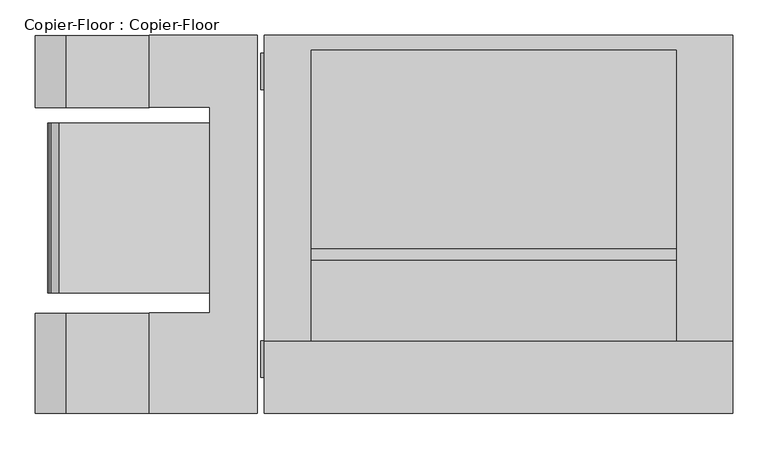
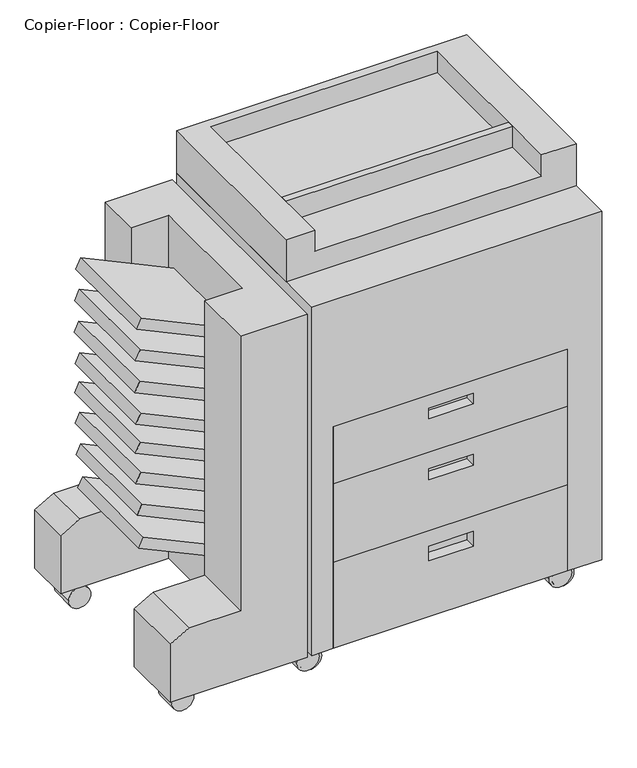
"""IFC4 building model written with IfcOpenShell, lengths in millimetres: proxy geometry, Copier-Floor : Copier-Floor."""

from ifc_helpers import new_model, si_unit, point, frame, frame_2d, origin, place, context, project, spatial, polyline, circle_curve, trimmed, segment, composite_curve, outline, extrude, faceted_brep, source, transform, mapped, element, save


def copier_floor_copier_floor_8d74970a(model_context):
    return source(origin(), model_context, "Body", "SolidModel", [
        extrude(outline(polyline([(358.0987222, -618.0517332), (335.0785044, -628.7862371), (232.9041289, -409.6725817), (260.929928, -409.6725817), (358.0987222, -618.0517332)])), frame((0.0, -72.1685532, 0.0), z_axis=(0.0, 1.0, 0.0), x_axis=(0.0, 0.0, 1.0)), (0.0, 0.0, 1.0), 239.8222339),
        extrude(outline(polyline([(438.9521671, -622.0116402), (415.9319493, -632.7461441), (311.9110388, -409.6725817), (339.9368379, -409.6725817), (438.9521671, -622.0116402)])), frame((0.0, -72.1685532, 0.0), z_axis=(0.0, 1.0, 0.0), x_axis=(0.0, 0.0, 1.0)), (0.0, 0.0, 1.0), 239.8222339),
        extrude(outline(polyline([(516.4459532, -624.7861736), (493.4257355, -635.5206775), (388.1110388, -409.6725817), (416.1368379, -409.6725817), (516.4459532, -624.7861736)])), frame((0.0, -72.1685532, 0.0), z_axis=(0.0, 1.0, 0.0), x_axis=(0.0, 0.0, 1.0)), (0.0, 0.0, 1.0), 239.8222339),
        extrude(outline(polyline([(811.8732774, -625.5671218), (788.8530596, -636.3016256), (683.1742009, -409.6725817), (711.2, -409.6725817), (811.8732774, -625.5671218)])), frame((0.0, -72.1685532, 0.0), z_axis=(0.0, 1.0, 0.0), x_axis=(0.0, 0.0, 1.0)), (0.0, 0.0, 1.0), 239.8222339),
        extrude(outline(polyline([(589.7121876, -625.7577903), (566.6919698, -636.4922942), (460.9242009, -409.6725817), (488.95, -409.6725817), (589.7121876, -625.7577903)])), frame((0.0, -72.1685532, 0.0), z_axis=(0.0, 1.0, 0.0), x_axis=(0.0, 0.0, 1.0)), (0.0, 0.0, 1.0), 239.8222339),
        extrude(outline(polyline([(659.0988749, -624.7642131), (636.0786571, -635.4987169), (530.7742009, -409.6725817), (558.8, -409.6725817), (659.0988749, -624.7642131)])), frame((0.0, -72.1685532, 0.0), z_axis=(0.0, 1.0, 0.0), x_axis=(0.0, 0.0, 1.0)), (0.0, 0.0, 1.0), 239.8222339),
        extrude(outline(polyline([(736.3657716, -627.0521803), (713.3455538, -637.7866841), (606.9742009, -409.6725817), (635.0, -409.6725817), (736.3657716, -627.0521803)])), frame((0.0, -72.1685532, 0.0), z_axis=(0.0, 1.0, 0.0), x_axis=(0.0, 0.0, 1.0)), (0.0, 0.0, 1.0), 239.8222339),
        faceted_brep([(-655.4522418, -242.0310532, 76.2), (-342.5743224, -242.0310532, 76.2), (-342.5743224, -242.0310532, 901.7), (-494.9743224, -242.0310532, 901.7), (-494.9743224, -242.0310532, 241.3), (-612.1273026, -242.0310532, 241.3), (-655.4522418, -242.0310532, 216.2863347), (-655.4522418, 291.3689468, 76.2), (-655.4522418, 291.3689468, 216.2863347), (-612.1273026, 291.3689468, 241.3), (-494.9743224, 291.3689468, 241.3), (-494.9743224, 291.3689468, 901.7), (-342.5743224, 291.3689468, 901.7), (-342.5743224, 291.3689468, 76.2), (-655.4522418, -100.8888364, 76.2), (-409.6725817, -100.8888364, 76.2), (-409.6725817, 189.7689468, 76.2), (-655.4522418, 189.7689468, 76.2), (-494.9743224, 189.7689468, 901.7), (-409.6725817, 189.7689468, 901.7), (-409.6725817, -100.8888364, 901.7), (-494.9743224, -100.8888364, 901.7), (-494.9743224, -100.8888364, 241.3), (-494.9743224, 189.7689468, 241.3), (-612.1273026, -100.8888364, 241.3), (-612.1273026, 189.7689468, 241.3), (-655.4522418, -100.8888364, 216.2863347), (-655.4522418, 189.7689468, 216.2863347)], [[[0, 1, 2, 3, 4, 5, 6]], [[7, 8, 9, 10, 11, 12, 13]], [[1, 0, 14, 15, 16, 17, 7, 13]], [[2, 1, 13, 12]], [[3, 2, 12, 11, 18, 19, 20, 21]], [[4, 3, 21, 22]], [[11, 10, 23, 18]], [[5, 4, 22, 24]], [[10, 9, 25, 23]], [[6, 5, 24, 26]], [[9, 8, 27, 25]], [[0, 6, 26, 14]], [[8, 7, 17, 27]], [[16, 19, 18, 23, 25, 27, 17]], [[20, 15, 14, 26, 24, 22, 21]], [[19, 16, 15, 20]]]),
        faceted_brep([(249.314028, -242.0310532, 472.3553727), (249.314028, -242.0310532, 609.6), (-284.085972, -242.0310532, 609.6), (-284.085972, -242.0310532, 472.3553727), (-66.7741493, -242.0310532, 578.8591447), (34.8258507, -242.0310532, 578.8591447), (34.8258507, -242.0310532, 553.4591447), (-66.7741493, -242.0310532, 553.4591447), (249.314028, -191.2310532, 472.3553727), (-284.085972, -191.2310532, 472.3553727), (-284.085972, -191.2310532, 609.6), (249.314028, -191.2310532, 609.6), (34.8258507, -216.6310532, 578.8591447), (-66.7741493, -216.6310532, 578.8591447), (-66.7741493, -216.6310532, 553.4591447), (34.8258507, -216.6310532, 553.4591447)], [[[0, 1, 2, 3], [4, 5, 6, 7]], [[8, 9, 10, 11]], [[1, 0, 8, 11]], [[2, 1, 11, 10]], [[3, 2, 10, 9]], [[0, 3, 9, 8]], [[12, 13, 14, 15]], [[13, 12, 5, 4]], [[14, 13, 4, 7]], [[15, 14, 7, 6]], [[12, 15, 6, 5]]]),
        faceted_brep([(249.314028, -242.0310532, 283.8723489), (249.314028, -242.0310532, 472.3553727), (-284.085972, -242.0310532, 472.3553727), (-284.085972, -242.0310532, 283.8723489), (-66.7741493, -242.0310532, 432.3774172), (34.8258507, -242.0310532, 432.3774172), (34.8258507, -242.0310532, 406.4), (-66.7741493, -242.0310532, 406.4), (249.314028, -191.2310532, 283.8723489), (-284.085972, -191.2310532, 283.8723489), (-284.085972, -191.2310532, 472.3553727), (249.314028, -191.2310532, 472.3553727), (34.8258507, -216.6310532, 432.3774172), (-66.7741493, -216.6310532, 432.3774172), (-66.7741493, -216.6310532, 406.4), (34.8258507, -216.6310532, 406.4)], [[[0, 1, 2, 3], [4, 5, 6, 7]], [[8, 9, 10, 11]], [[1, 0, 8, 11]], [[2, 1, 11, 10]], [[3, 2, 10, 9]], [[0, 3, 9, 8]], [[12, 13, 14, 15]], [[13, 12, 5, 4]], [[14, 13, 4, 7]], [[15, 14, 7, 6]], [[12, 15, 6, 5]]]),
        faceted_brep([(249.314028, -242.0310532, 76.2), (249.314028, -242.0310532, 283.8723489), (-284.085972, -242.0310532, 283.8723489), (-284.085972, -242.0310532, 76.2), (-66.7741493, -242.0310532, 246.5423898), (34.8258507, -242.0310532, 246.5423898), (34.8258507, -242.0310532, 211.1096445), (-66.7741493, -242.0310532, 211.1096445), (249.314028, -191.2310532, 76.2), (-284.085972, -191.2310532, 76.2), (-284.085972, -191.2310532, 283.8723489), (249.314028, -191.2310532, 283.8723489), (34.8258507, -216.6310532, 246.5423898), (-66.7741493, -216.6310532, 246.5423898), (-66.7741493, -216.6310532, 211.1096445), (34.8258507, -216.6310532, 211.1096445)], [[[0, 1, 2, 3], [4, 5, 6, 7]], [[8, 9, 10, 11]], [[1, 0, 8, 11]], [[2, 1, 11, 10]], [[3, 2, 10, 9]], [[0, 3, 9, 8]], [[12, 13, 14, 15]], [[13, 12, 5, 4]], [[14, 13, 4, 7]], [[15, 14, 7, 6]], [[12, 15, 6, 5]]]),
        faceted_brep([(328.0345418, 291.3689468, 1016.0), (-332.3654582, 291.3689468, 1016.0), (-332.3654582, -139.9052479, 1016.0), (-267.2959958, -139.9052479, 1016.0), (-267.2959958, 271.1108348, 1016.0), (249.314028, 271.1108348, 1016.0), (249.314028, -139.9052479, 1016.0), (328.0345418, -139.9052479, 1016.0), (328.0345418, 291.3689468, 914.4), (328.0345418, -139.9052479, 914.4), (-332.3654582, -139.9052479, 914.4), (-332.3654582, 291.3689468, 914.4), (249.314028, -139.9052479, 965.2), (-267.2959958, -139.9052479, 965.2), (249.314028, 271.1108348, 965.2), (-267.2959958, 271.1108348, 965.2)], [[[0, 1, 2, 3, 4, 5, 6, 7]], [[8, 9, 10, 11]], [[1, 0, 8, 11]], [[2, 1, 11, 10]], [[10, 9, 7, 6, 12, 13, 3, 2]], [[0, 7, 9, 8]], [[14, 15, 13, 12]], [[15, 14, 5, 4]], [[13, 15, 4, 3]], [[14, 12, 6, 5]]]),
        faceted_brep([(328.0345418, 291.3689468, 914.4), (-332.3654582, 291.3689468, 914.4), (-332.3654582, -242.0310532, 914.4), (328.0345418, -242.0310532, 914.4), (328.0345418, 291.3689468, 76.2), (328.0345418, -242.0310532, 76.2), (249.314028, -242.0310532, 76.2), (249.314028, -191.2310532, 76.2), (-284.085972, -191.2310532, 76.2), (-284.085972, -242.0310532, 76.2), (-332.3654582, -242.0310532, 76.2), (-332.3654582, 291.3689468, 76.2), (-284.085972, -242.0310532, 609.6), (249.314028, -242.0310532, 609.6), (-284.085972, -191.2310532, 609.6), (249.314028, -191.2310532, 609.6)], [[[0, 1, 2, 3]], [[4, 5, 6, 7, 8, 9, 10, 11]], [[1, 0, 4, 11]], [[2, 1, 11, 10]], [[3, 2, 10, 9, 12, 13, 6, 5]], [[0, 3, 5, 4]], [[14, 8, 7, 15]], [[8, 14, 12, 9]], [[15, 7, 6, 13]], [[14, 15, 13, 12]]]),
        extrude(outline(polyline([(886.7027049, -622.6279196), (863.6824871, -633.3624234), (759.3742009, -409.6725817), (787.4, -409.6725817), (886.7027049, -622.6279196)])), frame((0.0, -72.1685532, 0.0), z_axis=(0.0, 1.0, 0.0), x_axis=(0.0, 0.0, 1.0)), (0.0, 0.0, 1.0), 239.8222339),
        extrude(outline(composite_curve([segment(trimmed(circle_curve(frame_2d((31.7967794, -597.2732438)), 25.4), [point((31.7967794, -622.6732438))], [point((31.7967794, -571.8732438))], False, "CARTESIAN"), True, "CONTINUOUS"), segment(trimmed(circle_curve(frame_2d((31.7967794, -597.2732438)), 25.4), [point((31.7967794, -571.8732438))], [point((31.7967794, -622.6732438))], False, "CARTESIAN"), True, "CONTINUOUS")], self_intersect=False)), frame((0.0, 215.1689468, 0.0), z_axis=(0.0, 1.0, 0.0), x_axis=(0.0, 0.0, 1.0)), (0.0, 0.0, 1.0), 55.9418879),
        extrude(outline(composite_curve([segment(trimmed(circle_curve(frame_2d((31.7967794, -597.2732438)), 25.4), [point((31.7967794, -622.6732438))], [point((31.7967794, -571.8732438))], False, "CARTESIAN"), True, "CONTINUOUS"), segment(trimmed(circle_curve(frame_2d((31.7967794, -597.2732438)), 25.4), [point((31.7967794, -571.8732438))], [point((31.7967794, -622.6732438))], False, "CARTESIAN"), True, "CONTINUOUS")], self_intersect=False)), frame((0.0, -191.2310532, 0.0), z_axis=(0.0, 1.0, 0.0), x_axis=(0.0, 0.0, 1.0)), (0.0, 0.0, 1.0), 51.3258053),
        extrude(outline(composite_curve([segment(trimmed(circle_curve(frame_2d((27.9129458, -312.2555429)), 25.4), [point((27.9129458, -337.6555429))], [point((27.9129458, -286.8555429))], False, "CARTESIAN"), True, "CONTINUOUS"), segment(trimmed(circle_curve(frame_2d((27.9129458, -312.2555429)), 25.4), [point((27.9129458, -286.8555429))], [point((27.9129458, -337.6555429))], False, "CARTESIAN"), True, "CONTINUOUS")], self_intersect=False)), frame((0.0, 215.1689468, 0.0), z_axis=(0.0, 1.0, 0.0), x_axis=(0.0, 0.0, 1.0)), (0.0, 0.0, 1.0), 51.3258053),
        extrude(outline(composite_curve([segment(trimmed(circle_curve(frame_2d((27.9129458, 262.7398948)), 25.4), [point((27.9129458, 237.3398948))], [point((27.9129458, 288.1398948))], False, "CARTESIAN"), True, "CONTINUOUS"), segment(trimmed(circle_curve(frame_2d((27.9129458, 262.7398948)), 25.4), [point((27.9129458, 288.1398948))], [point((27.9129458, 237.3398948))], False, "CARTESIAN"), True, "CONTINUOUS")], self_intersect=False)), frame((0.0, 215.1689468, 0.0), z_axis=(0.0, 1.0, 0.0), x_axis=(0.0, 0.0, 1.0)), (0.0, 0.0, 1.0), 51.3258053),
        extrude(outline(composite_curve([segment(trimmed(circle_curve(frame_2d((27.9129458, -312.2555429)), 25.4), [point((27.9129458, -337.6555429))], [point((27.9129458, -286.8555429))], False, "CARTESIAN"), True, "CONTINUOUS"), segment(trimmed(circle_curve(frame_2d((27.9129458, -312.2555429)), 25.4), [point((27.9129458, -286.8555429))], [point((27.9129458, -337.6555429))], False, "CARTESIAN"), True, "CONTINUOUS")], self_intersect=False)), frame((0.0, -191.2310532, 0.0), z_axis=(0.0, 1.0, 0.0), x_axis=(0.0, 0.0, 1.0)), (0.0, 0.0, 1.0), 51.3258053),
        extrude(outline(composite_curve([segment(trimmed(circle_curve(frame_2d((27.9129458, 262.7398948)), 25.4), [point((27.9129458, 237.3398948))], [point((27.9129458, 288.1398948))], False, "CARTESIAN"), True, "CONTINUOUS"), segment(trimmed(circle_curve(frame_2d((27.9129458, 262.7398948)), 25.4), [point((27.9129458, 288.1398948))], [point((27.9129458, 237.3398948))], False, "CARTESIAN"), True, "CONTINUOUS")], self_intersect=False)), frame((0.0, -191.2310532, 0.0), z_axis=(0.0, 1.0, 0.0), x_axis=(0.0, 0.0, 1.0)), (0.0, 0.0, 1.0), 51.3258053),
        extrude(outline(composite_curve([segment(trimmed(circle_curve(frame_2d((27.9129458, -306.6302391)), 25.4), [point((27.9129458, -332.0302391))], [point((27.9129458, -281.2302391))], False, "CARTESIAN"), True, "CONTINUOUS"), segment(trimmed(circle_curve(frame_2d((27.9129458, -306.6302391)), 25.4), [point((27.9129458, -281.2302391))], [point((27.9129458, -332.0302391))], False, "CARTESIAN"), True, "CONTINUOUS")], self_intersect=False)), frame((0.0, -191.2310532, 0.0), z_axis=(0.0, 1.0, 0.0), x_axis=(0.0, 0.0, 1.0)), (0.0, 0.0, 1.0), 51.3258053),
        extrude(outline(composite_curve([segment(trimmed(circle_curve(frame_2d((27.9129458, 268.3651986)), 25.4), [point((27.9129458, 242.9651986))], [point((27.9129458, 293.7651986))], False, "CARTESIAN"), True, "CONTINUOUS"), segment(trimmed(circle_curve(frame_2d((27.9129458, 268.3651986)), 25.4), [point((27.9129458, 293.7651986))], [point((27.9129458, 242.9651986))], False, "CARTESIAN"), True, "CONTINUOUS")], self_intersect=False)), frame((0.0, -191.2310532, 0.0), z_axis=(0.0, 1.0, 0.0), x_axis=(0.0, 0.0, 1.0)), (0.0, 0.0, 1.0), 51.3258053),
        extrude(outline(polyline([(249.314028, -26.1310532), (-267.2959958, -26.1310532), (-267.2959958, -10.0577181), (249.314028, -10.0577181), (249.314028, -26.1310532)])), frame((0.0, 0.0, 965.2), z_axis=(0.0, 0.0, 1.0), x_axis=(1.0, 0.0, 0.0)), (0.0, 0.0, 1.0), 50.8),
    ])


if __name__ == "__main__":
    model = new_model("IFC4")
    model_context = context("Model", 3, world=origin())
    ifc_project = project(units=[si_unit("LENGTHUNIT", "METRE", prefix="MILLI")], contexts=[model_context])
    site = spatial("IfcSite", under=ifc_project)
    building = spatial("IfcBuilding", under=site)
    placement = place(None, origin())
    copier_floor_copier_floor_shape = copier_floor_copier_floor_8d74970a(model_context)
    element("IfcBuildingElementProxy", 1, Name="Copier-Floor : Copier-Floor", ObjectType="Copier-Floor : Copier-Floor", at=placement, inside=building, context=model_context, shape_type="MappedRepresentation", body=[
        mapped(copier_floor_copier_floor_shape, transform((0.0, 0.0, 0.0), x_axis=(1.0, 0.0, 0.0), y_axis=(0.0, 1.0, 0.0), z_axis=(0.0, 0.0, 1.0))),
    ])
    save(model, "model.ifc")

# Revit data of these elements
# Type "Copier-Floor : Copier-Floor"
#   Assembly Code = "E1010800"
# Element 1 (IfcBuildingElementProxy, "Copier-Floor : Copier-Floor")
#   Materials on its faces: "Plastic - White", "Plastic - Gray,Dark"
# Materials
#   "Plastic - White": class "Plastic", colour RGB 255 255 255, transparency 0, Cost = 0
#   "Plastic - Gray,Dark": class "Plastic", colour RGB 255 255 255, transparency 0, Cost = 0
